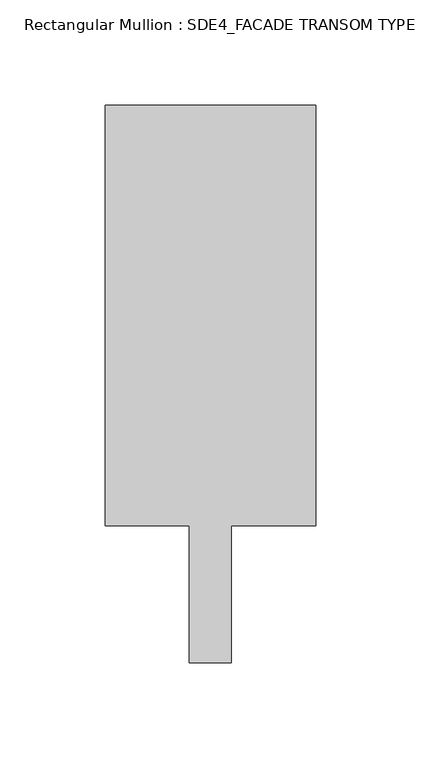
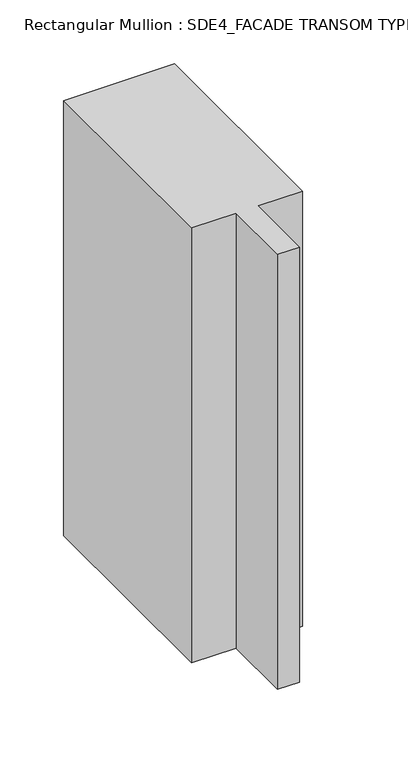
"""IFC4 building model written with IfcOpenShell, lengths in millimetres: member geometry, Rectangular Mullion : SDE4_FACADE TRANSOM TYPE 2."""

from ifc_helpers import new_model, si_unit, frame, origin, place, context, project, spatial, polyline, outline, extrude, source, transform, mapped, element, save


def rectangular_mullion_sde4_facade_transom_type_2_5e272fec(model_context):
    return source(origin(), model_context, "Body", "SweptSolid", [
        extrude(outline(polyline([(50.0, 132.5), (50.0, -67.5), (10.0, -67.5), (10.0, -132.5), (-10.0, -132.5), (-10.0, -67.5), (-50.0, -67.5), (-50.0, 132.5), (50.0, 132.5)])), frame((0.0, 0.0, -415.0002218), z_axis=(0.0, 0.0, 1.0), x_axis=(1.0, 0.0, 0.0)), (0.0, 0.0, 1.0), 415.0002218),
    ])


if __name__ == "__main__":
    model = new_model("IFC4")
    model_context = context("Model", 3, world=origin())
    ifc_project = project(units=[si_unit("LENGTHUNIT", "METRE", prefix="MILLI")], contexts=[model_context])
    site = spatial("IfcSite", under=ifc_project)
    building = spatial("IfcBuilding", under=site)
    placement = place(None, origin())
    rectangular_mullion_sde4_facade_transom_type_2_shape = rectangular_mullion_sde4_facade_transom_type_2_5e272fec(model_context)
    element("IfcMember", 1, ObjectType="Rectangular Mullion : SDE4_FACADE TRANSOM TYPE 2", at=placement, inside=building, context=model_context, shape_type="MappedRepresentation", body=[
        mapped(rectangular_mullion_sde4_facade_transom_type_2_shape, transform((0.0, 0.0, 0.0), x_axis=(1.0, 0.0, 0.0), y_axis=(0.0, 1.0, 0.0), z_axis=(0.0, 0.0, 1.0))),
    ])
    save(model, "model.ifc")

# Revit data of these elements
# Type "Rectangular Mullion : SDE4_FACADE TRANSOM TYPE 2"
#   built-in parameter 1007322 = 0.869423 (stored number, unit not read)
#   built-in parameter 1007321 = 0.164042 (stored number, unit not read)
#   built-in parameter 1007320 = 0.164042 (stored number, unit not read)
